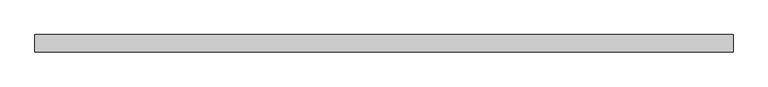
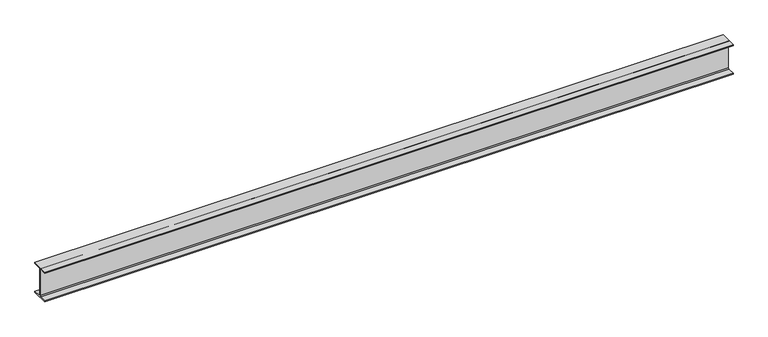
"""IFC4 building model written with IfcOpenShell, lengths in millimetres: beam geometry, Old_Steel Beam_H-KSD3502 : H_SB_ASB_H-400×200x8x13."""

from ifc_helpers import new_model, si_unit, point, frame, frame_2d, origin, place, context, project, spatial, polyline, circle_curve, trimmed, segment, composite_curve, outline, extrude, source, transform, mapped, element, save


def beam_e3027ac9(model_context):
    return source(origin(), model_context, "Body", "SweptSolid", [
        extrude(outline(composite_curve([segment(polyline([(82.5, -141.5), (82.5, -151.7), (-82.5, -151.7), (-82.5, -141.5), (-11.9, -141.5)]), True, "CONTINUOUS"), segment(trimmed(circle_curve(frame_2d((-11.9, -132.6)), 8.9), [point((-11.9, -141.5))], [point((-3.0, -132.6))], True, "CARTESIAN"), True, "CONTINUOUS"), segment(polyline([(-3.0, -132.6), (-3.0, 132.6)]), True, "CONTINUOUS"), segment(trimmed(circle_curve(frame_2d((-11.9, 132.6)), 8.9), [point((-3.0, 132.6))], [point((-11.9, 141.5))], True, "CARTESIAN"), True, "CONTINUOUS"), segment(polyline([(-11.9, 141.5), (-82.5, 141.5), (-82.5, 151.7), (82.5, 151.7), (82.5, 141.5), (11.9, 141.5)]), True, "CONTINUOUS"), segment(trimmed(circle_curve(frame_2d((11.9, 132.6)), 8.9), [point((11.9, 141.5))], [point((3.0, 132.6))], True, "CARTESIAN"), True, "CONTINUOUS"), segment(polyline([(3.0, 132.6), (3.0, -132.6)]), True, "CONTINUOUS"), segment(trimmed(circle_curve(frame_2d((11.9, -132.6)), 8.9), [point((3.0, -132.6))], [point((11.9, -141.5))], True, "CARTESIAN"), True, "CONTINUOUS"), segment(polyline([(11.9, -141.5), (82.5, -141.5)]), True, "CONTINUOUS")], self_intersect=False)), frame((-3244.5360727, 0.0, 0.0), z_axis=(1.0, 0.0, 0.0), x_axis=(0.0, 1.0, 0.0)), (0.0, 0.0, 1.0), 6649.3360727),
    ])


if __name__ == "__main__":
    model = new_model("IFC4")
    model_context = context("Model", 3, world=origin())
    ifc_project = project(units=[si_unit("LENGTHUNIT", "METRE", prefix="MILLI")], contexts=[model_context])
    site = spatial("IfcSite", under=ifc_project)
    building = spatial("IfcBuilding", under=site)
    placement = place(None, origin())
    beam_shape = beam_e3027ac9(model_context)
    element("IfcBeam", 1, ObjectType="Old_Steel Beam_H-KSD3502 : H_SB_ASB_H-400×200x8x13", at=placement, inside=building, context=model_context, shape_type="MappedRepresentation", body=[
        mapped(beam_shape, transform((0.0, 0.0, 0.0), x_axis=(1.0, 0.0, 0.0), y_axis=(0.0, 1.0, 0.0), z_axis=(0.0, 0.0, 1.0))),
    ])
    save(model, "model.ifc")

# Revit data of these elements
# Type "Old_Steel Beam_H-KSD3502 : H_SB_ASB_H-400×200x8x13"
#   Width = 20.0 cm
#   Web Thickness = 0.8 cm
#   Web Fillet = 1.6 cm
#   Warping Constant = 648999.0 cm⁶
#   Torsional Moment of Inertia = 35.8981 cm⁴
#   Torsional Modulus = 1.0 cm³
#   Section Area = 84.12 cm²
#   Plastic Modulus weak axis = 268.0 cm³
#   Plastic Modulus strong axis = 1330.0 cm³
#   Perimeter = 1.56 m²/m
#   Nominal Weight = 66.00 kgf/m
#   Moment of Inertia weak axis = 1740.00 cm⁴
#   Moment of Inertia strong axis = 23700.00 cm⁴
#   Height = 40.0 cm
#   Flange Thickness = 1.3 cm
#   Elastic Modulus weak axis = 174.0 cm³
#   Elastic Modulus strong axis = 1190.0 cm³
#   Centroid Vertical = 20.0 cm
#   Centroid Horizontal = 10.0 cm
#   Length [instance default] = 1.5240 m
#   Structural Material [instance default] = Steel, 45-345
#   Assembly Code = ""
# Element 1 (IfcBeam, "Old_Steel Beam_H-KSD3502 : H_SB_ASB_H-400×200x8x13")
#   Structural Material = none
# Materials
#   "Steel, 45-345": class "Metal", colour RGB 189 187 185, transparency 0, Description = "Steel 345 MPa", Cost = 0
